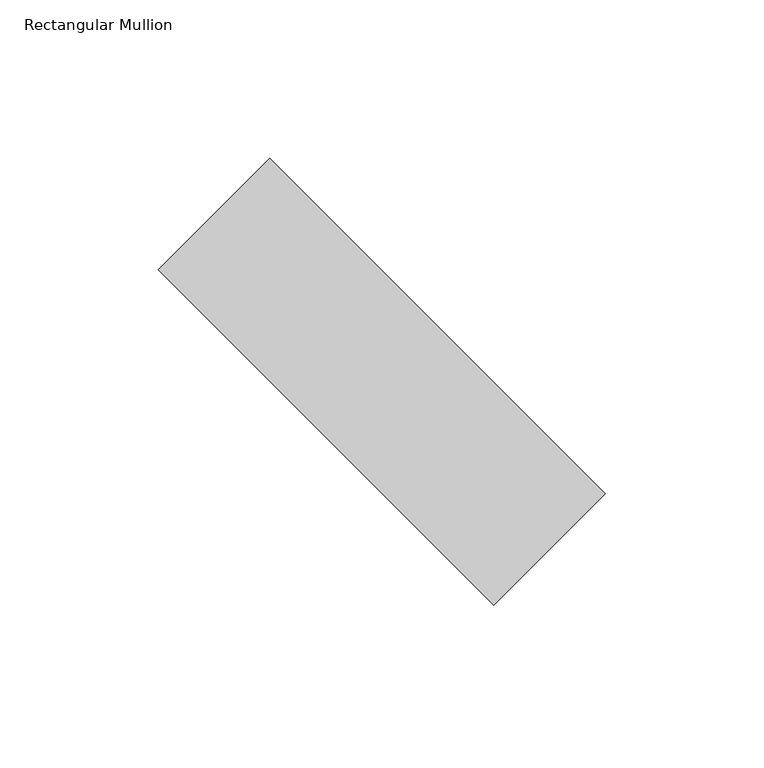
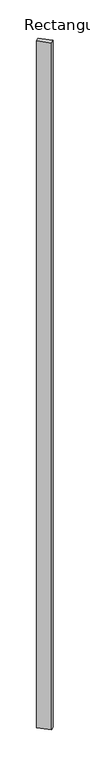
"""IFC4 building model written with IfcOpenShell, lengths in millimetres: member geometry, Rectangular Mullion : tilted mullions."""

import ifcopenshell
import ifcopenshell.guid

model = None  # the IFC model being written
_history = None  # IfcOwnerHistory: only IFC2X3 demands one
_inside = {}  # id of a spatial element -> (the spatial element, [elements in it])
_under = {}  # id of a project, library or spatial element -> (it, [spatial elements below it])
_declared = {}  # id of a project -> (the project, [libraries it declares])
_typed = {}  # id of a type object -> (the type object, [elements of that type])
_made_of = {}  # id of a material, layer set ... -> (it, [elements and type objects made of it])


def new_model(schema):
    """Start an empty IFC model of exactly this schema.

    Asked for "IFC4X3", IfcOpenShell would pick the latest addendum, in which some entities
    have other attributes; the version numbers below select the first issue.
    IFC2X3 requires an IfcOwnerHistory on every rooted entity: one is made here for all.
    """
    global model, _history
    if schema == "IFC4X3":
        model = ifcopenshell.file(schema_version=(4, 3, 0, 0))
    else:
        model = ifcopenshell.file(schema=schema)
    _inside.clear()
    _under.clear()
    _declared.clear()
    _typed.clear()
    _made_of.clear()
    _history = None
    if model.schema == "IFC2X3":
        org = make("IfcOrganization", Name="unknown")
        user = make(
            "IfcPersonAndOrganization",
            ThePerson=make("IfcPerson", FamilyName="unknown"),
            TheOrganization=org,
        )
        app = make(
            "IfcApplication",
            ApplicationDeveloper=org,
            Version="unknown",
            ApplicationFullName="unknown",
            ApplicationIdentifier="unknown",
        )
        _history = make(
            "IfcOwnerHistory",
            OwningUser=user,
            OwningApplication=app,
            ChangeAction="ADDED",
            CreationDate=0,
        )
    return model


def make(cls, **values):
    """One entity of the class cls with the attributes given. An attribute that is None is left unset."""
    return model.create_entity(
        cls, **{name: value for name, value in values.items() if value is not None}
    )


def rooted(cls, **values):
    """An entity with a GlobalId (a new one), such as an element, a storey or a relation."""
    return make(cls, GlobalId=ifcopenshell.guid.new(), OwnerHistory=_history, **values)


def si_unit(unit_type, name, prefix=None):
    """IfcSIUnit, for example si_unit("LENGTHUNIT", "METRE", prefix="MILLI")."""
    return make("IfcSIUnit", UnitType=unit_type, Prefix=prefix, Name=name)


def assignment(units):
    """IfcUnitAssignment: the units of a project."""
    return None if units is None else make("IfcUnitAssignment", Units=units)


def point(xyz):
    """IfcCartesianPoint."""
    return None if xyz is None else make("IfcCartesianPoint", Coordinates=xyz)


def direction(xyz):
    """IfcDirection."""
    return None if xyz is None else make("IfcDirection", DirectionRatios=xyz)


def frame(location, z_axis=None, x_axis=None):
    """IfcAxis2Placement3D, a coordinate frame: its origin and axes. An axis left out is left unset."""
    return make(
        "IfcAxis2Placement3D",
        Location=point(location),
        Axis=direction(z_axis),
        RefDirection=direction(x_axis),
    )


def origin():
    """The frame at (0, 0, 0) with its axes left unset."""
    return frame((0.0, 0.0, 0.0))


def place(relative_to, where):
    """IfcLocalPlacement: puts the frame where relative to a parent placement (None: the world)."""
    return make(
        "IfcLocalPlacement", PlacementRelTo=relative_to, RelativePlacement=where
    )


def context(
    kind, dimensions, precision=None, world=None, true_north=None, identifier=None
):
    """IfcGeometricRepresentationContext, for example the 3D "Model" context."""
    return make(
        "IfcGeometricRepresentationContext",
        ContextIdentifier=identifier,
        ContextType=kind,
        CoordinateSpaceDimension=dimensions,
        Precision=precision,
        WorldCoordinateSystem=world,
        TrueNorth=true_north,
    )


def project(units=None, contexts=None):
    """IfcProject with its units and contexts."""
    return rooted(
        "IfcProject",
        Name="project",
        RepresentationContexts=contexts,
        UnitsInContext=assignment(units),
    )


def spatial(cls, under=None, at=None, **own):
    """A site, building, storey or space (cls), placed at a placement, below another one or the project."""
    s = rooted(cls, ObjectPlacement=at, **own)
    if under is not None:
        _under.setdefault(under.id(), (under, []))[1].append(s)
    return s


def polyline(points):
    """IfcPolyline through the points."""
    return make("IfcPolyline", Points=[point(p) for p in points])


def outline(outer, holes=None, kind="AREA"):
    """IfcArbitraryClosedProfileDef: a profile drawn as a closed curve; with holes, ...WithVoids."""
    if holes is None:
        return make("IfcArbitraryClosedProfileDef", ProfileType=kind, OuterCurve=outer)
    return make(
        "IfcArbitraryProfileDefWithVoids",
        ProfileType=kind,
        OuterCurve=outer,
        InnerCurves=holes,
    )


def extrude(swept, where, along, depth):
    """IfcExtrudedAreaSolid: the profile swept, set in the frame where, extruded along a direction by depth."""
    return make(
        "IfcExtrudedAreaSolid",
        SweptArea=swept,
        Position=where,
        ExtrudedDirection=direction(along),
        Depth=depth,
    )


def shape(context_of_items, identifier, shape_type, items):
    """IfcShapeRepresentation: the items that make up one representation, for example the "Body"."""
    return make(
        "IfcShapeRepresentation",
        ContextOfItems=context_of_items,
        RepresentationIdentifier=identifier,
        RepresentationType=shape_type,
        Items=items,
    )


def source(mapping_origin, context_of_items, identifier, shape_type, items):
    """IfcRepresentationMap: a shape defined once, which mapped items show again and again."""
    return make(
        "IfcRepresentationMap",
        MappingOrigin=mapping_origin,
        MappedRepresentation=shape(context_of_items, identifier, shape_type, items),
    )


def transform(
    local_origin,
    x_axis=None,
    y_axis=None,
    z_axis=None,
    scale=None,
    scale2=None,
    scale3=None,
    uniform=True,
):
    """IfcCartesianTransformationOperator3D, or its non-uniform kind. x_axis, y_axis, z_axis: its Axis1, 2, 3."""
    if uniform:
        return make(
            "IfcCartesianTransformationOperator3D",
            Axis1=direction(x_axis),
            Axis2=direction(y_axis),
            LocalOrigin=point(local_origin),
            Scale=scale,
            Axis3=direction(z_axis),
        )
    return make(
        "IfcCartesianTransformationOperator3DnonUniform",
        Axis1=direction(x_axis),
        Axis2=direction(y_axis),
        LocalOrigin=point(local_origin),
        Scale=scale,
        Axis3=direction(z_axis),
        Scale2=scale2,
        Scale3=scale3,
    )


def mapped(mapping_source, mapping_target):
    """IfcMappedItem: shows the shape of a source again, moved by a transform."""
    return make(
        "IfcMappedItem", MappingSource=mapping_source, MappingTarget=mapping_target
    )


def made_of(thing, what):
    """Note that an element or type object is made of a material, layer set ...; save() writes the relation."""
    if what is not None:
        _made_of.setdefault(what.id(), (what, []))[1].append(thing)
    return thing


def element(
    cls,
    number,
    at=None,
    inside=None,
    cuts=None,
    type_object=None,
    material=None,
    context=None,
    identifier="Body",
    shape_type=None,
    held_by="IfcProductDefinitionShape",
    body=None,
    shapes=None,
    **own,
):
    """One element of the class cls, such as IfcWall. Its Tag is "e" and its number.

    at: its placement. inside: the storey or other place that contains it. cuts: it is an
    opening in that element (IfcRelVoidsElement). A single representation is given by context,
    identifier, shape_type and body (its items); several are given by shapes. held_by: the class
    of the entity that holds the representations. save() writes the other relations.
    """
    e = rooted(cls, Tag="e%d" % number, ObjectPlacement=at, **own)
    if body is not None:
        shapes = [shape(context, identifier, shape_type, body)]
    if shapes is not None:
        e.Representation = make(held_by, Representations=shapes)
    if inside is not None:
        _inside.setdefault(inside.id(), (inside, []))[1].append(e)
    if cuts is not None:
        rooted(
            "IfcRelVoidsElement", RelatingBuildingElement=cuts, RelatedOpeningElement=e
        )
    if type_object is not None:
        _typed.setdefault(type_object.id(), (type_object, []))[1].append(e)
    return made_of(e, material)


def aggregate(whole, parts):
    """IfcRelAggregates: a whole, such as a stair, and the parts it consists of."""
    return rooted("IfcRelAggregates", RelatingObject=whole, RelatedObjects=parts)


def save(model, path):
    """Write the relations noted so far, then the file.

    IfcRelAggregates (storeys below a building ...), IfcRelContainedInSpatialStructure (elements
    in a storey), IfcRelDefinesByType, IfcRelAssociatesMaterial and IfcRelDeclares: one each for
    every whole, place, type object, material and project.
    """
    for whole, parts in _under.values():
        aggregate(whole, parts)
    for where, things in _inside.values():
        rooted(
            "IfcRelContainedInSpatialStructure",
            RelatedElements=things,
            RelatingStructure=where,
        )
    for kind, things in _typed.values():
        rooted("IfcRelDefinesByType", RelatedObjects=things, RelatingType=kind)
    for what, things in _made_of.values():
        rooted("IfcRelAssociatesMaterial", RelatedObjects=things, RelatingMaterial=what)
    for by, libraries in _declared.values():
        rooted("IfcRelDeclares", RelatingContext=by, RelatedDefinitions=libraries)
    model.write(path)


def rectangular_mullion_5ffb7332(model_context):
    return source(origin(), model_context, "Body", "SweptSolid", [
        extrude(outline(polyline([(-35.3553391, 70.7106781), (70.7106781, -35.3553391), (35.3553391, -70.7106781), (-70.7106781, 35.3553391), (-35.3553391, 70.7106781)])), frame((0.0, 0.0, -7999.4864286), z_axis=(0.0, 0.0, 1.0), x_axis=(1.0, 0.0, 0.0)), (0.0, 0.0, 1.0), 7999.4864286),
    ])


if __name__ == "__main__":
    model = new_model("IFC4")
    model_context = context("Model", 3, world=origin())
    ifc_project = project(units=[si_unit("LENGTHUNIT", "METRE", prefix="MILLI")], contexts=[model_context])
    site = spatial("IfcSite", under=ifc_project)
    building = spatial("IfcBuilding", under=site)
    placement = place(None, origin())
    rectangular_mullion_shape = rectangular_mullion_5ffb7332(model_context)
    element("IfcMember", 1, ObjectType="Rectangular Mullion : tilted mullions", at=placement, inside=building, context=model_context, shape_type="MappedRepresentation", body=[
        mapped(rectangular_mullion_shape, transform((0.0, 0.0, 0.0), x_axis=(1.0, 0.0, 0.0), y_axis=(0.0, 1.0, 0.0), z_axis=(0.0, 0.0, 1.0))),
    ])
    save(model, "model.ifc")

# Revit data of these elements
# Type "Rectangular Mullion : tilted mullions"
#   built-in parameter 1007304 = 0.492126 (stored number, unit not read)
#   built-in parameter 1007301 = 0.082021 (stored number, unit not read)
#   built-in parameter 1007300 = 0.082021 (stored number, unit not read)
# Element 1 (IfcMember, "Rectangular Mullion : tilted mullions")
#   Materials on its faces: "Aluminum"
# Materials
#   "Aluminum": class "Metal", colour RGB 244 244 244, transparency 0, Description = "Aluminum 6061", Cost = 0
